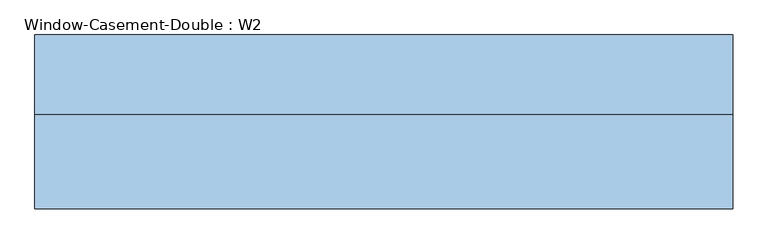
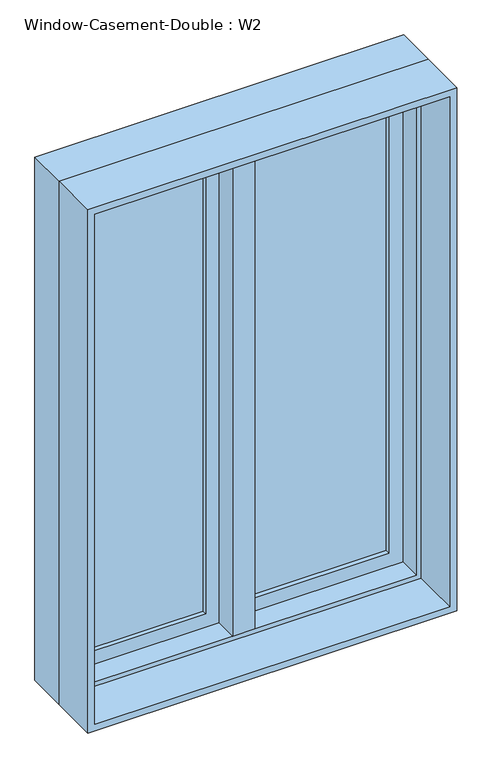
"""IFC4 building model written with IfcOpenShell, lengths in millimetres: window geometry, Window-Casement-Double : W2."""

from ifc_helpers import new_model, si_unit, frame, origin, place, context, project, spatial, polyline, outline, extrude, faceted_brep, source, transform, mapped, element, save


def window_casement_double_w2_71d7abdb(model_context):
    return source(origin(), model_context, "Body", "SolidModel", [
        faceted_brep([(9.525, 134.05, 2401.7), (-9.525, 134.05, 2401.7), (-9.525, 83.25, 2401.7), (9.525, 83.25, 2401.7), (9.525, 134.05, 927.1), (9.525, 83.25, 927.1), (-9.525, 83.25, 927.1), (-9.525, 134.05, 927.1), (-9.525, 83.25, 946.15), (-9.525, 83.25, 2382.65), (-30.1625, 83.25, 946.15), (-30.1625, 83.25, 2382.65), (-30.1625, 19.75, 946.15), (-30.1625, 19.75, 2382.65), (30.1625, 19.75, 946.15), (30.1625, 19.75, 2382.65), (30.1625, 83.25, 946.15), (30.1625, 83.25, 2382.65), (9.525, 83.25, 946.15), (9.525, 83.25, 2382.65)], [[[0, 1, 2, 3]], [[4, 5, 6, 7]], [[1, 0, 4, 7]], [[2, 1, 7, 6, 8, 9]], [[9, 8, 10, 11]], [[11, 10, 12, 13]], [[13, 12, 14, 15]], [[15, 14, 16, 17]], [[17, 16, 18, 19]], [[0, 3, 19, 18, 5, 4]], [[18, 8, 6, 5]], [[9, 19, 3, 2]], [[8, 18, 16, 14, 12, 10]], [[19, 9, 11, 13, 15, 17]]]),
        extrude(outline(polyline([(-66.675, 115.0), (-66.675, 108.65), (-430.15, 108.65), (-430.15, 115.0), (-66.675, 115.0)])), frame((0.0, 0.0, 984.25), z_axis=(0.0, 0.0, 1.0), x_axis=(1.0, 0.0, 0.0)), (0.0, 0.0, 1.0), 1360.3),
        extrude(outline(polyline([(-430.15, 95.95), (-430.15, 102.3), (-66.675, 102.3), (-66.675, 95.95), (-430.15, 95.95)])), frame((0.0, 0.0, 984.25), z_axis=(0.0, 0.0, 1.0), x_axis=(1.0, 0.0, 0.0)), (0.0, 0.0, 1.0), 1360.3),
        extrude(outline(polyline([(430.15, 115.0), (430.15, 108.65), (66.675, 108.65), (66.675, 115.0), (430.15, 115.0)])), frame((0.0, 0.0, 984.25), z_axis=(0.0, 0.0, 1.0), x_axis=(1.0, 0.0, 0.0)), (0.0, 0.0, 1.0), 1360.3),
        extrude(outline(polyline([(66.675, 95.95), (66.675, 102.3), (430.15, 102.3), (430.15, 95.95), (66.675, 95.95)])), frame((0.0, 0.0, 984.25), z_axis=(0.0, 0.0, 1.0), x_axis=(1.0, 0.0, 0.0)), (0.0, 0.0, 1.0), 1360.3),
        extrude(outline(polyline([(2401.7, -487.3), (927.1, -487.3), (927.1, -9.525), (2401.7, -9.525), (2401.7, -487.3)]), holes=[polyline([(2344.55, -66.675), (984.25, -66.675), (984.25, -430.15), (2344.55, -430.15), (2344.55, -66.675)])]), frame((0.0, 83.25, 0.0), z_axis=(0.0, 1.0, 0.0), x_axis=(0.0, 0.0, 1.0)), (0.0, 0.0, 1.0), 44.45),
        extrude(outline(polyline([(927.1, 487.3), (2401.7, 487.3), (2401.7, 9.525), (927.1, 9.525), (927.1, 487.3)]), holes=[polyline([(984.25, 66.675), (2344.55, 66.675), (2344.55, 430.15), (984.25, 430.15), (984.25, 66.675)])]), frame((0.0, 83.25, 0.0), z_axis=(0.0, 1.0, 0.0), x_axis=(0.0, 0.0, 1.0)), (0.0, 0.0, 1.0), 44.45),
        extrude(outline(polyline([(2414.4, -500.0), (914.4, -500.0), (914.4, 500.0), (2414.4, 500.0), (2414.4, -500.0)]), holes=[polyline([(2395.35, 480.95), (933.45, 480.95), (933.45, -480.95), (2395.35, -480.95), (2395.35, 480.95)])]), frame((0.0, -115.0, 0.0), z_axis=(0.0, 1.0, 0.0), x_axis=(0.0, 0.0, 1.0)), (0.0, 0.0, 1.0), 134.75),
        faceted_brep([(468.25, 83.25, 2382.65), (468.25, 19.75, 2382.65), (-468.25, 19.75, 2382.65), (-468.25, 83.25, 2382.65), (487.3, 134.05, 2401.7), (487.3, 83.25, 2401.7), (-487.3, 83.25, 2401.7), (-487.3, 134.05, 2401.7), (500.0, 19.75, 2414.4), (500.0, 134.05, 2414.4), (-500.0, 134.05, 2414.4), (-500.0, 19.75, 2414.4), (-468.25, 19.75, 946.15), (-468.25, 83.25, 946.15), (-487.3, 83.25, 927.1), (-487.3, 134.05, 927.1), (-500.0, 134.05, 914.4), (-500.0, 19.75, 914.4), (468.25, 19.75, 946.15), (468.25, 83.25, 946.15), (487.3, 83.25, 927.1), (487.3, 134.05, 927.1), (500.0, 134.05, 914.4), (500.0, 19.75, 914.4)], [[[0, 1, 2, 3]], [[4, 5, 6, 7]], [[8, 9, 10, 11]], [[3, 2, 12, 13]], [[7, 6, 14, 15]], [[11, 10, 16, 17]], [[13, 12, 18, 19]], [[15, 14, 20, 21]], [[17, 16, 22, 23]], [[11, 17, 23, 8], [1, 18, 12, 2]], [[19, 18, 1, 0]], [[5, 20, 14, 6], [3, 13, 19, 0]], [[21, 20, 5, 4]], [[23, 22, 9, 8]], [[9, 22, 16, 10], [7, 15, 21, 4]]]),
    ])


if __name__ == "__main__":
    model = new_model("IFC4")
    model_context = context("Model", 3, world=origin())
    ifc_project = project(units=[si_unit("LENGTHUNIT", "METRE", prefix="MILLI")], contexts=[model_context])
    site = spatial("IfcSite", under=ifc_project)
    building = spatial("IfcBuilding", under=site)
    placement = place(None, origin())
    window_casement_double_w2_shape = window_casement_double_w2_71d7abdb(model_context)
    element("IfcWindow", 1, ObjectType="Window-Casement-Double : W2", at=placement, inside=building, context=model_context, shape_type="MappedRepresentation", body=[
        mapped(window_casement_double_w2_shape, transform((0.0, 0.0, 0.0), x_axis=(1.0, 0.0, 0.0), y_axis=(0.0, 1.0, 0.0), z_axis=(0.0, 0.0, 1.0))),
    ])
    save(model, "model.ifc")

# Revit data of these elements
# Type "Window-Casement-Double : W2"
#   Type Mark = "28"
#   Fire Rating = "0.5h"
#   Assembly Code = "B2020100"
#   Analytic Construction = "Double glazing - domestic"
#   Frame Extension [instance default] = 0.00635 m
#   Window Inset [instance default] = 0 m
#   Wall Thickness [instance default] = 0.1524 m
#   Interior Wall Closure [instance default] = 0.05715 m
#   Half Width = 0.5 m
#   Visual Light Transmittance = 0.81
#   Thermal Resistance (R) = 0.319569 (m²·K)/W
#   Solar Heat Gain Coefficient = 0.76
#   Rough Width = 1.0127 m
#   Rough Height = 1.5127 m
#   Height = 1.5 m
#   Heat Transfer Coefficient (U) = 3.12929 W/(m²·K)
#   Exterior Wall Closure [instance default] = 0.03175 m
#   Extension Jamb [instance default] = 0.05715 m
#   Default Sill Height = 0.9144 m
#   Width = 1 m
#   Muntin Visibility = yes
#   Interior Trim Visibility [instance default] = yes
#   Exterior Trim Visibility [instance default] = yes
#   Extension Jamb Visibility [instance default] = yes
#   Interior Trim Material = Wood - Stained
#   Muntin Pattern = Muntin Pattern_2x2 : Muntin Pattern_2x2
#   Interior Trim = Trim-Window-Interior-Flat : Picture Frame
#   Interior Frame Material = Wood - Stained
#   Glass Panel Material = Glass
#   Exterior Trim Material = Clad - White
#   Exterior Trim = Trim-Window-Exterior-Flat : with Sill
#   Exterior Frame Material = Clad - White
#   Wall Closure = (empty or 0)
# Element 1 (IfcWindow, "Window-Casement-Double : W2")
#   Wall Thickness = 0.23 m
#   Extension Jamb = 0.13475 m
#   Materials on its faces: "Wood - Stained", "Glass", "Clad - White"
# Materials
#   "Wood - Stained": class "Wood", colour RGB 224 178 126, transparency 0, Cost = 0
#   "Glass": class "Glass", colour RGB 0 128 192, transparency 0.9, Description = "Soda Lime Glass", Cost = 0
#   "Clad - White": class "Wood", colour RGB 242 242 238, transparency 0, Cost = 0
